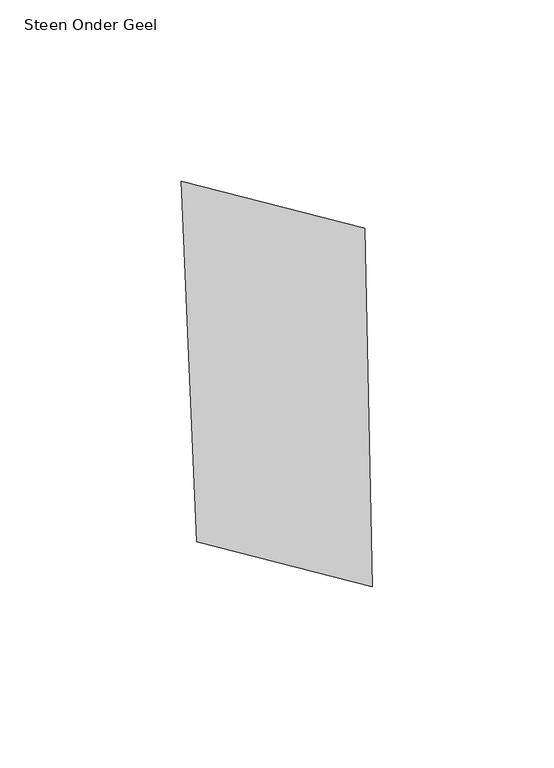
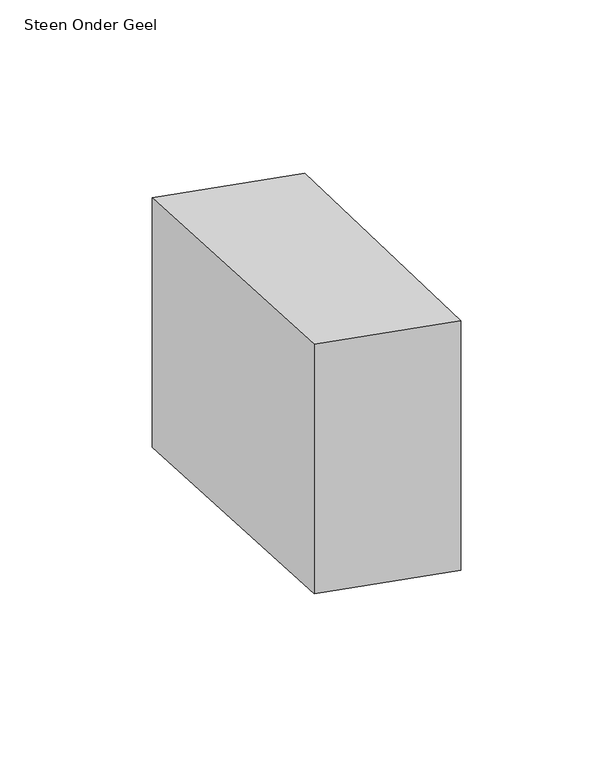
"""IFC4 building model written with IfcOpenShell, lengths in millimetres: proxy geometry, 00_GMA_steen_versie_4 : Steen Onder Geel."""

from ifc_helpers import new_model, si_unit, origin, origin_with_axes, place, context, project, spatial, polyline, outline, extrude, source, transform, mapped, element, save


def steen_onder_geel_ebb1c59a(model_context):
    return source(origin(), model_context, "Body", "SweptSolid", [
        extrude(outline(polyline([(99.7053594, 116.7158033), (101.8182033, 17.9498507), (53.3670387, 30.2983181), (49.2021739, 129.6118979), (99.7053594, 116.7158033)])), origin_with_axes(), (0.0, 0.0, 1.0), 100.0),
    ])


if __name__ == "__main__":
    model = new_model("IFC4")
    model_context = context("Model", 3, world=origin())
    ifc_project = project(units=[si_unit("LENGTHUNIT", "METRE", prefix="MILLI")], contexts=[model_context])
    site = spatial("IfcSite", under=ifc_project)
    building = spatial("IfcBuilding", under=site)
    placement = place(None, origin())
    steen_onder_geel_shape = steen_onder_geel_ebb1c59a(model_context)
    element("IfcBuildingElementProxy", 1, Name="00_GMA_steen_versie_4 : Steen Onder Geel", ObjectType="00_GMA_steen_versie_4 : Steen Onder Geel", at=placement, inside=building, context=model_context, shape_type="MappedRepresentation", body=[
        mapped(steen_onder_geel_shape, transform((0.0, 0.0, 0.0), x_axis=(1.0, 0.0, 0.0), y_axis=(0.0, 1.0, 0.0), z_axis=(0.0, 0.0, 1.0))),
    ])
    save(model, "model.ifc")

# Revit data of these elements
# Type "00_GMA_steen_versie_4 : Steen Onder Geel"
#   StootVoegHalfBoven [instance default] = 5 mm
#   StootVoegHalf [instance default] = 5 mm
#   StootVoegBreedteOnder = 10 mm
#   StootVoegBreedteBoven = 10 mm
#   Steendikte = 100 mm
#   LintVoegOnderHalf = 0 mm
#   LintVoegOnder = 0 mm
#   LintVoegBovenHalf = 5 mm
#   LintVoegBoven = 10 mm
#   materiaal = 21_steen_geel
#   MateriaalVoeg = none
#   Default Elevation = 0
# Element 1 (IfcBuildingElementProxy, "00_GMA_steen_versie_4 : Steen Onder Geel")
#   Materials on its faces: "21_steen_geel"
# Materials
#   "21_steen_geel": class "Unassigned", colour RGB 202 202 0, transparency 0, Cost = 0
